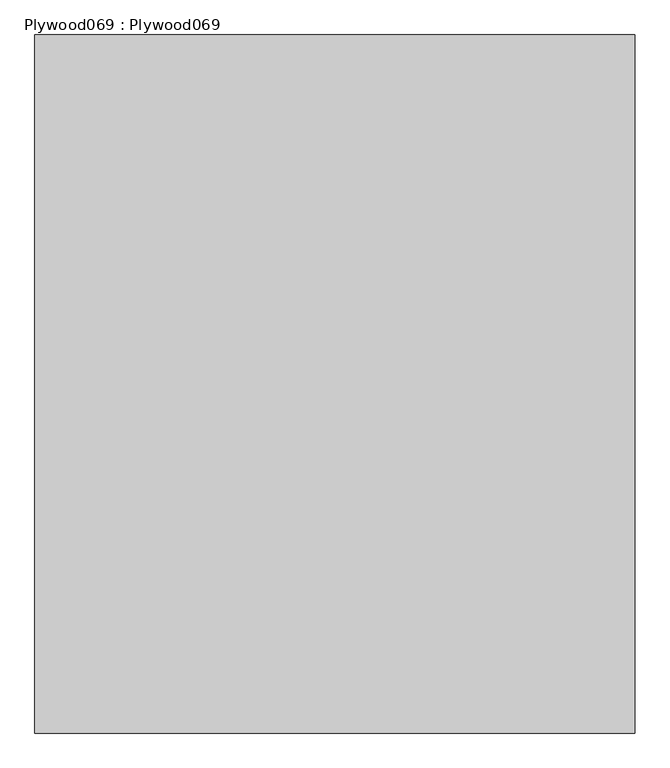
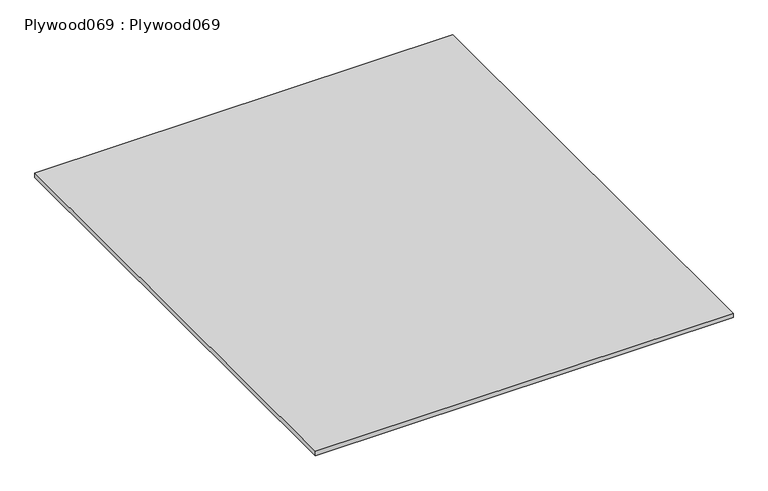
"""IFC4 building model written with IfcOpenShell, lengths in millimetres: proxy geometry, Plywood069 : Plywood069."""

from ifc_helpers import new_model, si_unit, frame, origin, place, context, project, spatial, polyline, outline, extrude, source, transform, mapped, element, save


def plywood069_plywood069_31ddffa7(model_context):
    return source(origin(), model_context, "Body", "SweptSolid", [
        extrude(outline(polyline([(-5503.7121051, 7982.1531721), (-7223.1276325, 7982.1531721), (-7223.1276325, 9982.1531721), (-5503.7121051, 9982.1531721), (-5503.7121051, 7982.1531721)])), frame((0.0, 0.0, 39934.8960083), z_axis=(0.0, 0.0, 1.0), x_axis=(1.0, 0.0, 0.0)), (0.0, 0.0, 1.0), 19.05),
    ])


if __name__ == "__main__":
    model = new_model("IFC4")
    model_context = context("Model", 3, world=origin())
    ifc_project = project(units=[si_unit("LENGTHUNIT", "METRE", prefix="MILLI")], contexts=[model_context])
    site = spatial("IfcSite", under=ifc_project)
    building = spatial("IfcBuilding", under=site)
    placement = place(None, origin())
    plywood069_plywood069_shape = plywood069_plywood069_31ddffa7(model_context)
    element("IfcBuildingElementProxy", 1, Name="Plywood069 : Plywood069", ObjectType="Plywood069 : Plywood069", at=placement, inside=building, context=model_context, shape_type="MappedRepresentation", body=[
        mapped(plywood069_plywood069_shape, transform((0.0, 0.0, 0.0), x_axis=(1.0, 0.0, 0.0), y_axis=(0.0, 1.0, 0.0), z_axis=(0.0, 0.0, 1.0))),
    ])
    save(model, "model.ifc")

# Revit data of these elements
# Type "Plywood069 : Plywood069"
#   NameOverride = "Plywood069"
# Element 1 (IfcBuildingElementProxy, "Plywood069 : Plywood069")
#   Materials on its faces: "CDX PLYWOOD -  SEE STRUCTURAL DWGS"
# Materials
#   "CDX PLYWOOD -  SEE STRUCTURAL DWGS": class "Unassigned", colour RGB 177 130 114, transparency 0, Cost = 0
